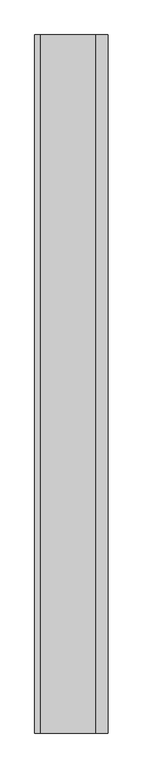
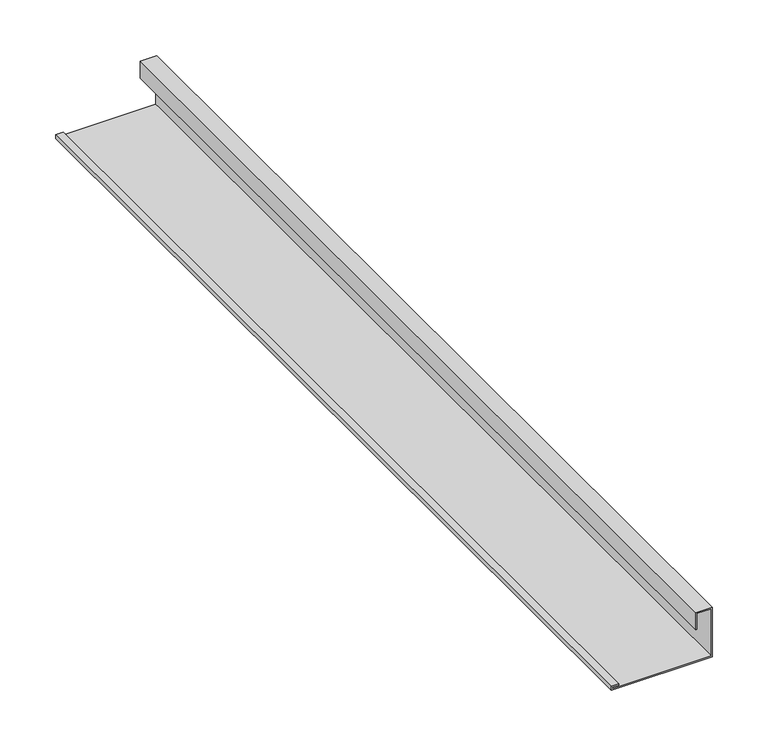
"""IFC4 building model written with IfcOpenShell, lengths in millimetres: proxy geometry, RECEIVER TRIM001 : RECEIVER TRIM001."""

from ifc_helpers import new_model, si_unit, frame, origin, place, context, project, spatial, polyline, outline, extrude, source, transform, mapped, element, save


def generic_models_bb0b6a77(model_context):
    return source(origin(), model_context, "Body", "SweptSolid", [
        extrude(outline(polyline([(42632.0615589, 6031.5496814), (42613.2870495, 6031.5496814), (42613.2870495, 6032.7403064), (42630.8709339, 6032.7403064), (42630.8709339, 6047.6002567), (42578.8995464, 6047.6002567), (42578.8995464, 5944.8903428), (42580.5523621, 5944.8903428), (42580.5523621, 5951.5825651), (42581.7429871, 5951.5825651), (42581.7429871, 5943.6997178), (42577.7089214, 5943.6997178), (42577.7089214, 6048.7908817), (42632.0615589, 6048.7908817), (42632.0615589, 6031.5496814)])), frame((0.0, -1052.8906574, 0.0), z_axis=(0.0, 1.0, 0.0), x_axis=(0.0, 0.0, 1.0)), (0.0, 0.0, 1.0), 1000.0),
    ])


if __name__ == "__main__":
    model = new_model("IFC4")
    model_context = context("Model", 3, world=origin())
    ifc_project = project(units=[si_unit("LENGTHUNIT", "METRE", prefix="MILLI")], contexts=[model_context])
    site = spatial("IfcSite", under=ifc_project)
    building = spatial("IfcBuilding", under=site)
    placement = place(None, origin())
    generic_models_shape = generic_models_bb0b6a77(model_context)
    element("IfcBuildingElementProxy", 1, Name="RECEIVER TRIM001 : RECEIVER TRIM001", ObjectType="RECEIVER TRIM001 : RECEIVER TRIM001", at=placement, inside=building, context=model_context, shape_type="MappedRepresentation", body=[
        mapped(generic_models_shape, transform((0.0, 0.0, 0.0), x_axis=(1.0, 0.0, 0.0), y_axis=(0.0, 1.0, 0.0), z_axis=(0.0, 0.0, 1.0))),
    ])
    save(model, "model.ifc")

# Revit data of these elements
# Type "RECEIVER TRIM001 : RECEIVER TRIM001"
#   NameOverride = "RECEIVER TRIM001"
# Element 1 (IfcBuildingElementProxy, "RECEIVER TRIM001 : RECEIVER TRIM001")
#   Materials on its faces: "RECEIVER TRIM"
# Materials
#   "RECEIVER TRIM": class "Unassigned", colour RGB 245 226 176, transparency 0, Cost = 0
